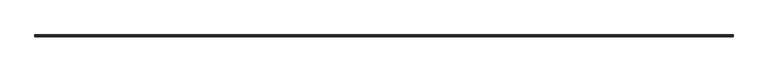
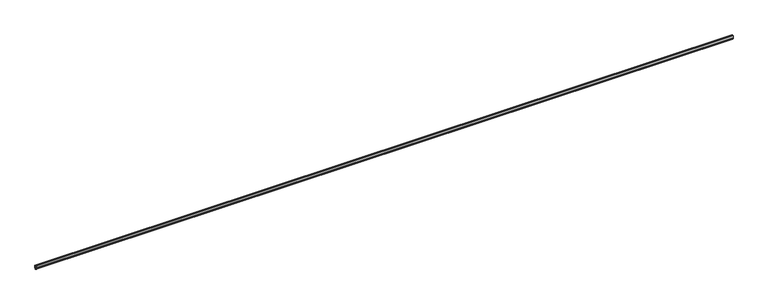
"""IFC4 building model written with IfcOpenShell, lengths in millimetres: proxy geometry, Generic Models 7:Generic Models 1:1:Generic Models 1:1 : Generic Models 7:Generic Models 1:337419:28 : Generic Models 7:Generic Models 1:1:Generic Models 1:1 : Generic Models 7:Generic Models 1:337419:306201."""

from ifc_helpers import new_model, si_unit, frame, origin, place, context, project, spatial, polyline, outline, extrude, source, transform, mapped, element, save


def generic_models_5d2521c6(model_context):
    return source(origin(), model_context, "Body", "SweptSolid", [
        extrude(outline(polyline([(-578873.6913841, -11.7361843), (-578874.4640193, -10.0156223), (-578876.6309901, -7.396472), (-578879.3314857, -6.195765), (-578882.1430382, -6.6013407), (-578884.6258064, -8.5497508), (-578886.3913841, -11.7361843), (-578886.3913841, 0.0), (-578884.4598576, -0.7548172), (-578880.0413841, -1.3821894), (-578875.6229105, -0.7548172), (-578873.6913841, 0.0), (-578873.6913841, -11.7361843)])), frame((591280.6367239, 0.0, 0.0), z_axis=(1.0, 0.0, 0.0), x_axis=(0.0, 1.0, 0.0)), (0.0, 0.0, 1.0), 4782.0596551),
        extrude(outline(polyline([(-578873.8505919, -18.5829513), (-578875.0767542, -22.4021798), (-578877.2862223, -25.0451679), (-578880.0413841, -25.9884394), (-578882.7965458, -25.0451679), (-578885.006014, -22.4021798), (-578886.2321763, -18.5829513), (-578886.3913841, -16.4634394), (-578886.2321763, -14.3439275), (-578885.006014, -10.524699), (-578882.7965458, -7.8817109), (-578880.0413841, -6.9384394), (-578877.2862223, -7.8817109), (-578875.0767542, -10.524699), (-578873.8505919, -14.3439275), (-578873.6913841, -16.4634394), (-578873.8505919, -18.5829513)])), frame((591280.6367239, 0.0, 0.0), z_axis=(1.0, 0.0, 0.0), x_axis=(0.0, 1.0, 0.0)), (0.0, 0.0, 1.0), 4782.0596551),
    ])


if __name__ == "__main__":
    model = new_model("IFC4")
    model_context = context("Model", 3, world=origin())
    ifc_project = project(units=[si_unit("LENGTHUNIT", "METRE", prefix="MILLI")], contexts=[model_context])
    site = spatial("IfcSite", under=ifc_project)
    building = spatial("IfcBuilding", under=site)
    placement = place(None, origin())
    generic_models_shape = generic_models_5d2521c6(model_context)
    element("IfcBuildingElementProxy", 1, Name="Generic Models 7:Generic Models 1:1:Generic Models 1:1 : Generic Models 7:Generic Models 1:337419:28 : Generic Models 7:Generic Models 1:1:Generic Models 1:1 : Generic Models 7:Generic Models 1:337419:306201", ObjectType="Generic Models 7:Generic Models 1:1:Generic Models 1:1 : Generic Models 7:Generic Models 1:337419:28 : Generic Models 7:Generic Models 1:1:Generic Models 1:1 : Generic Models 7:Generic Models 1:337419:306201", at=placement, inside=building, context=model_context, shape_type="MappedRepresentation", body=[
        mapped(generic_models_shape, transform((0.0, 0.0, 0.0), x_axis=(1.0, 0.0, 0.0), y_axis=(0.0, 1.0, 0.0), z_axis=(0.0, 0.0, 1.0))),
    ])
    save(model, "model.ifc")

# Revit data of these elements
# Type "Generic Models 7:Generic Models 1:1:Generic Models 1:1 : Generic Models 7:Generic Models 1:337419:28 : Generic Models 7:Generic Models 1:1:Generic Models 1:1 : Generic Models 7:Generic Models 1:337419:306201"
#   NameOverride = "Generic Models 7:Generic Models 1:1:Generic Models 1:1 : Generic Models 7:Generic Models 1:337419:306201"
#   ObjectTypeOverride = "Generic Models 1:1 : Generic Models 7:Generic Models 1:337419"
#   Reference = "Generic Models 1"
#   Tag = "306201"
# Element 1 (IfcBuildingElementProxy, "Generic Models 7:Generic Models 1:1:Generic Models 1:1 : Generic Models 7:Generic Models 1:337419:28 : Generic Models 7:Generic Models 1:1:Generic Models 1:1 : Generic Models 7:Generic Models 1:337419:306201")
#   Materials on its faces: "SEMI-RIGID EPOXY SEALANT W/ BACKROD (REMOVE TEMP. JOINT FORM)"
# Materials
#   "SEMI-RIGID EPOXY SEALANT W/ BACKROD (REMOVE TEMP. JOINT FORM)": class "Unassigned", colour RGB 120 120 120, transparency 0, Cost = 0
